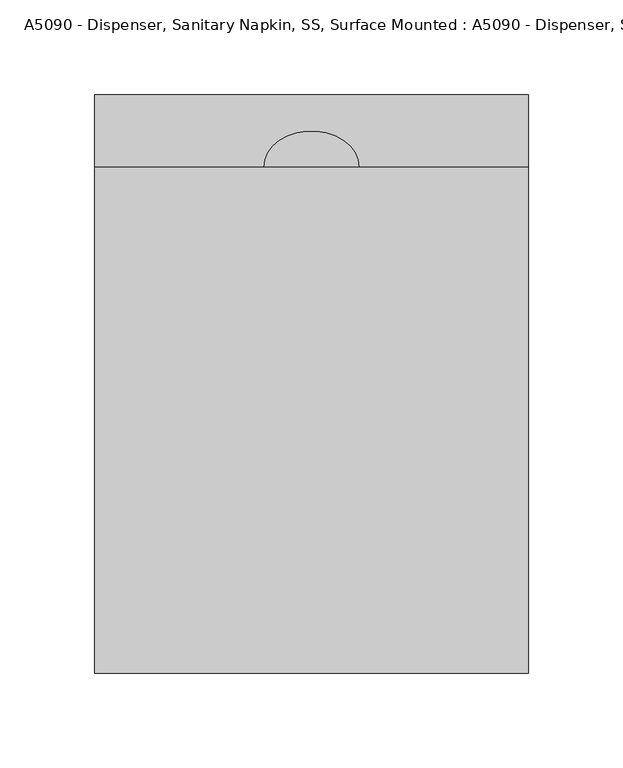
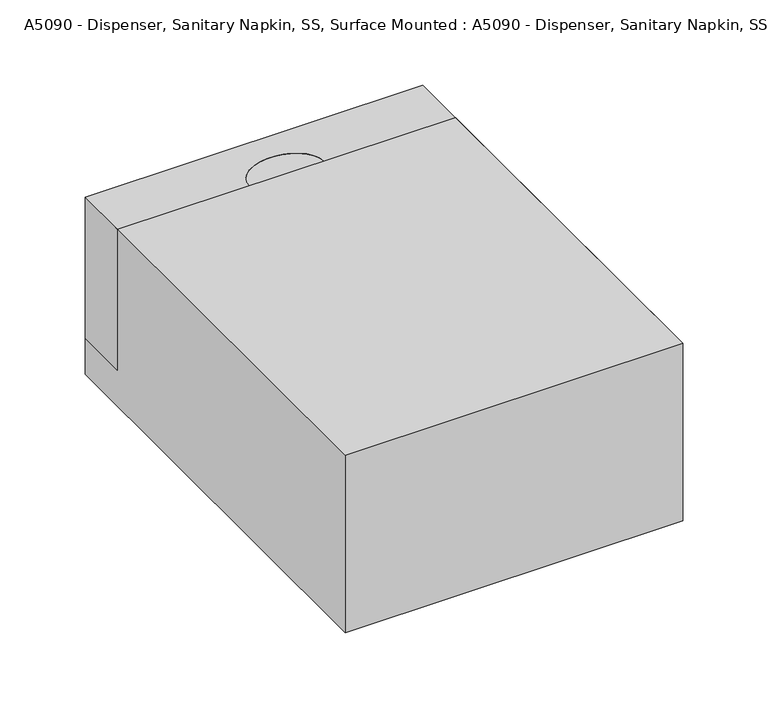
"""IFC4 building model written with IfcOpenShell, lengths in millimetres: proxy geometry, A5090 - Dispenser, Sanitary Napkin, SS, Surface Mounted : A5090 - Dispenser, Sanitary Napkin, SS, Surface Mounted."""

import ifcopenshell
import ifcopenshell.guid

model = None  # the IFC model being written
_history = None  # IfcOwnerHistory: only IFC2X3 demands one
_inside = {}  # id of a spatial element -> (the spatial element, [elements in it])
_under = {}  # id of a project, library or spatial element -> (it, [spatial elements below it])
_declared = {}  # id of a project -> (the project, [libraries it declares])
_typed = {}  # id of a type object -> (the type object, [elements of that type])
_made_of = {}  # id of a material, layer set ... -> (it, [elements and type objects made of it])


def new_model(schema):
    """Start an empty IFC model of exactly this schema.

    Asked for "IFC4X3", IfcOpenShell would pick the latest addendum, in which some entities
    have other attributes; the version numbers below select the first issue.
    IFC2X3 requires an IfcOwnerHistory on every rooted entity: one is made here for all.
    """
    global model, _history
    if schema == "IFC4X3":
        model = ifcopenshell.file(schema_version=(4, 3, 0, 0))
    else:
        model = ifcopenshell.file(schema=schema)
    _inside.clear()
    _under.clear()
    _declared.clear()
    _typed.clear()
    _made_of.clear()
    _history = None
    if model.schema == "IFC2X3":
        org = make("IfcOrganization", Name="unknown")
        user = make(
            "IfcPersonAndOrganization",
            ThePerson=make("IfcPerson", FamilyName="unknown"),
            TheOrganization=org,
        )
        app = make(
            "IfcApplication",
            ApplicationDeveloper=org,
            Version="unknown",
            ApplicationFullName="unknown",
            ApplicationIdentifier="unknown",
        )
        _history = make(
            "IfcOwnerHistory",
            OwningUser=user,
            OwningApplication=app,
            ChangeAction="ADDED",
            CreationDate=0,
        )
    return model


def make(cls, **values):
    """One entity of the class cls with the attributes given. An attribute that is None is left unset."""
    return model.create_entity(
        cls, **{name: value for name, value in values.items() if value is not None}
    )


def rooted(cls, **values):
    """An entity with a GlobalId (a new one), such as an element, a storey or a relation."""
    return make(cls, GlobalId=ifcopenshell.guid.new(), OwnerHistory=_history, **values)


def si_unit(unit_type, name, prefix=None):
    """IfcSIUnit, for example si_unit("LENGTHUNIT", "METRE", prefix="MILLI")."""
    return make("IfcSIUnit", UnitType=unit_type, Prefix=prefix, Name=name)


def assignment(units):
    """IfcUnitAssignment: the units of a project."""
    return None if units is None else make("IfcUnitAssignment", Units=units)


def point(xyz):
    """IfcCartesianPoint."""
    return None if xyz is None else make("IfcCartesianPoint", Coordinates=xyz)


def direction(xyz):
    """IfcDirection."""
    return None if xyz is None else make("IfcDirection", DirectionRatios=xyz)


def frame(location, z_axis=None, x_axis=None):
    """IfcAxis2Placement3D, a coordinate frame: its origin and axes. An axis left out is left unset."""
    return make(
        "IfcAxis2Placement3D",
        Location=point(location),
        Axis=direction(z_axis),
        RefDirection=direction(x_axis),
    )


def origin():
    """The frame at (0, 0, 0) with its axes left unset."""
    return frame((0.0, 0.0, 0.0))


def origin_with_axes():
    """The frame at (0, 0, 0) with the z axis (0, 0, 1) and the x axis (1, 0, 0) written out."""
    return frame((0.0, 0.0, 0.0), z_axis=(0.0, 0.0, 1.0), x_axis=(1.0, 0.0, 0.0))


def place(relative_to, where):
    """IfcLocalPlacement: puts the frame where relative to a parent placement (None: the world)."""
    return make(
        "IfcLocalPlacement", PlacementRelTo=relative_to, RelativePlacement=where
    )


def context(
    kind, dimensions, precision=None, world=None, true_north=None, identifier=None
):
    """IfcGeometricRepresentationContext, for example the 3D "Model" context."""
    return make(
        "IfcGeometricRepresentationContext",
        ContextIdentifier=identifier,
        ContextType=kind,
        CoordinateSpaceDimension=dimensions,
        Precision=precision,
        WorldCoordinateSystem=world,
        TrueNorth=true_north,
    )


def project(units=None, contexts=None):
    """IfcProject with its units and contexts."""
    return rooted(
        "IfcProject",
        Name="project",
        RepresentationContexts=contexts,
        UnitsInContext=assignment(units),
    )


def spatial(cls, under=None, at=None, **own):
    """A site, building, storey or space (cls), placed at a placement, below another one or the project."""
    s = rooted(cls, ObjectPlacement=at, **own)
    if under is not None:
        _under.setdefault(under.id(), (under, []))[1].append(s)
    return s


def polyline(points):
    """IfcPolyline through the points."""
    return make("IfcPolyline", Points=[point(p) for p in points])


def ellipse_curve(where, semi_axis1, semi_axis2):
    """IfcEllipse in the frame where."""
    return make(
        "IfcEllipse", Position=where, SemiAxis1=semi_axis1, SemiAxis2=semi_axis2
    )


def trimmed(basis, trim1, trim2, sense, master):
    """IfcTrimmedCurve: the piece of a basis curve between two trims."""
    return make(
        "IfcTrimmedCurve",
        BasisCurve=basis,
        Trim1=trim1,
        Trim2=trim2,
        SenseAgreement=sense,
        MasterRepresentation=master,
    )


def outline(outer, holes=None, kind="AREA"):
    """IfcArbitraryClosedProfileDef: a profile drawn as a closed curve; with holes, ...WithVoids."""
    if holes is None:
        return make("IfcArbitraryClosedProfileDef", ProfileType=kind, OuterCurve=outer)
    return make(
        "IfcArbitraryProfileDefWithVoids",
        ProfileType=kind,
        OuterCurve=outer,
        InnerCurves=holes,
    )


def extrude(swept, where, along, depth):
    """IfcExtrudedAreaSolid: the profile swept, set in the frame where, extruded along a direction by depth."""
    return make(
        "IfcExtrudedAreaSolid",
        SweptArea=swept,
        Position=where,
        ExtrudedDirection=direction(along),
        Depth=depth,
    )


def shape(context_of_items, identifier, shape_type, items):
    """IfcShapeRepresentation: the items that make up one representation, for example the "Body"."""
    return make(
        "IfcShapeRepresentation",
        ContextOfItems=context_of_items,
        RepresentationIdentifier=identifier,
        RepresentationType=shape_type,
        Items=items,
    )


def source(mapping_origin, context_of_items, identifier, shape_type, items):
    """IfcRepresentationMap: a shape defined once, which mapped items show again and again."""
    return make(
        "IfcRepresentationMap",
        MappingOrigin=mapping_origin,
        MappedRepresentation=shape(context_of_items, identifier, shape_type, items),
    )


def transform(
    local_origin,
    x_axis=None,
    y_axis=None,
    z_axis=None,
    scale=None,
    scale2=None,
    scale3=None,
    uniform=True,
):
    """IfcCartesianTransformationOperator3D, or its non-uniform kind. x_axis, y_axis, z_axis: its Axis1, 2, 3."""
    if uniform:
        return make(
            "IfcCartesianTransformationOperator3D",
            Axis1=direction(x_axis),
            Axis2=direction(y_axis),
            LocalOrigin=point(local_origin),
            Scale=scale,
            Axis3=direction(z_axis),
        )
    return make(
        "IfcCartesianTransformationOperator3DnonUniform",
        Axis1=direction(x_axis),
        Axis2=direction(y_axis),
        LocalOrigin=point(local_origin),
        Scale=scale,
        Axis3=direction(z_axis),
        Scale2=scale2,
        Scale3=scale3,
    )


def mapped(mapping_source, mapping_target):
    """IfcMappedItem: shows the shape of a source again, moved by a transform."""
    return make(
        "IfcMappedItem", MappingSource=mapping_source, MappingTarget=mapping_target
    )


def made_of(thing, what):
    """Note that an element or type object is made of a material, layer set ...; save() writes the relation."""
    if what is not None:
        _made_of.setdefault(what.id(), (what, []))[1].append(thing)
    return thing


def element(
    cls,
    number,
    at=None,
    inside=None,
    cuts=None,
    type_object=None,
    material=None,
    context=None,
    identifier="Body",
    shape_type=None,
    held_by="IfcProductDefinitionShape",
    body=None,
    shapes=None,
    **own,
):
    """One element of the class cls, such as IfcWall. Its Tag is "e" and its number.

    at: its placement. inside: the storey or other place that contains it. cuts: it is an
    opening in that element (IfcRelVoidsElement). A single representation is given by context,
    identifier, shape_type and body (its items); several are given by shapes. held_by: the class
    of the entity that holds the representations. save() writes the other relations.
    """
    e = rooted(cls, Tag="e%d" % number, ObjectPlacement=at, **own)
    if body is not None:
        shapes = [shape(context, identifier, shape_type, body)]
    if shapes is not None:
        e.Representation = make(held_by, Representations=shapes)
    if inside is not None:
        _inside.setdefault(inside.id(), (inside, []))[1].append(e)
    if cuts is not None:
        rooted(
            "IfcRelVoidsElement", RelatingBuildingElement=cuts, RelatedOpeningElement=e
        )
    if type_object is not None:
        _typed.setdefault(type_object.id(), (type_object, []))[1].append(e)
    return made_of(e, material)


def aggregate(whole, parts):
    """IfcRelAggregates: a whole, such as a stair, and the parts it consists of."""
    return rooted("IfcRelAggregates", RelatingObject=whole, RelatedObjects=parts)


def save(model, path):
    """Write the relations noted so far, then the file.

    IfcRelAggregates (storeys below a building ...), IfcRelContainedInSpatialStructure (elements
    in a storey), IfcRelDefinesByType, IfcRelAssociatesMaterial and IfcRelDeclares: one each for
    every whole, place, type object, material and project.
    """
    for whole, parts in _under.values():
        aggregate(whole, parts)
    for where, things in _inside.values():
        rooted(
            "IfcRelContainedInSpatialStructure",
            RelatedElements=things,
            RelatingStructure=where,
        )
    for kind, things in _typed.values():
        rooted("IfcRelDefinesByType", RelatedObjects=things, RelatingType=kind)
    for what, things in _made_of.values():
        rooted("IfcRelAssociatesMaterial", RelatedObjects=things, RelatingMaterial=what)
    for by, libraries in _declared.values():
        rooted("IfcRelDeclares", RelatingContext=by, RelatedDefinitions=libraries)
    model.write(path)


def plane_surface(at):
    """IfcPlane: the flat surface through the origin of the frame at, square to its z axis."""
    return make("IfcPlane", Position=at)


def extruded_surface(curve, direction_of_extrusion, depth):
    """IfcSurfaceOfLinearExtrusion: the curve pushed along a direction by depth."""
    return make(
        "IfcSurfaceOfLinearExtrusion",
        SweptCurve=make("IfcArbitraryOpenProfileDef", ProfileType="CURVE", Curve=curve),
        ExtrudedDirection=direction(direction_of_extrusion),
        Depth=depth,
    )


def advanced_brep(points, edges, surfaces, faces):
    """IfcAdvancedBrep: a solid bounded by faces that lie on surfaces and meet in shared edges.

    An edge is (start, end): straight between two places in points (the first is 0);
    or (start, end, curve); or (start, end, curve, False) where it runs against its curve.
    A face is (place in surfaces, loops), or (place, loops, False) where it looks against
    its surface's normal. A loop lists edges by number (the first is 1), with a minus sign
    where the edge is run from its end to its start. The first loop is the outer one.
    """
    corners = [point(p) for p in points]
    vertices = [make("IfcVertexPoint", VertexGeometry=c) for c in corners]
    made = []
    for start, end, *more in edges:
        made.append(
            make(
                "IfcEdgeCurve",
                EdgeStart=vertices[start],
                EdgeEnd=vertices[end],
                EdgeGeometry=more[0] if more else make("IfcPolyline", Points=[corners[start], corners[end]]),
                SameSense=more[1] if len(more) > 1 else True,
            )
        )
    hull = []
    for where, loops, *sense in faces:
        bounds = []
        for j, loop in enumerate(loops):
            ring = [make("IfcOrientedEdge", EdgeElement=made[abs(k) - 1], Orientation=k > 0) for k in loop]
            bounds.append(
                make(
                    "IfcFaceOuterBound" if j == 0 else "IfcFaceBound",
                    Bound=make("IfcEdgeLoop", EdgeList=ring),
                    Orientation=True,
                )
            )
        hull.append(make("IfcAdvancedFace", Bounds=bounds, FaceSurface=surfaces[where], SameSense=sense[0] if sense else True))
    return make("IfcAdvancedBrep", Outer=make("IfcClosedShell", CfsFaces=hull))


def a5090_dispenser_sanitary_napkin_ss_surface_mounted_a5090_ce8c1d57(model_context):
    return source(origin(), model_context, "Body", "SolidModel", [
        extrude(outline(polyline([(0.0, 127.0), (266.7, 127.0), (266.7, 25.4), (304.8, 25.4), (304.8, 0.0), (0.0, 0.0), (0.0, 127.0)])), frame((-114.3, 0.0, 0.0), z_axis=(1.0, 0.0, 0.0), x_axis=(0.0, 1.0, 0.0)), (0.0, 0.0, 1.0), 228.6),
        advanced_brep(
        [(114.3, 304.8, 127.0), (-114.3, 304.8, 127.0), (-114.3, 266.7, 127.0), (-25.4, 266.7, 127.0), (25.4, 266.7, 127.0), (114.3, 266.7, 127.0), (114.3, 304.8, 25.4), (114.3, 266.7, 25.4), (25.4, 266.7, 25.4), (-25.4, 266.7, 25.4), (-114.3, 266.7, 25.4), (-114.3, 304.8, 25.4)],
        [
            (0, 1),
            (1, 2),
            (2, 3),
            (3, 4, ellipse_curve(frame((0.0, 266.7, 127.0), z_axis=(0.0, 0.0, -1.0), x_axis=(1.0, 0.0, 0.0)), 25.4, 19.05)),
            (4, 5),
            (5, 0),
            (6, 7),
            (7, 8),
            (8, 9, ellipse_curve(frame((0.0, 266.7, 25.4), z_axis=(0.0, 0.0, 1.0), x_axis=(1.0, 0.0, 0.0)), 25.4, 19.05)),
            (9, 10),
            (10, 11),
            (11, 6),
            (0, 6),
            (11, 1),
            (10, 2),
            (9, 3),
            (8, 4),
            (7, 5),
        ],
        [
            plane_surface(frame((-114.3, 304.8, 127.0), z_axis=(0.0, 0.0, 1.0), x_axis=(-1.0, 0.0, 0.0))),
            plane_surface(frame((-114.3, 304.8, 25.4), z_axis=(0.0, 0.0, -1.0), x_axis=(1.0, 0.0, 0.0))),
            plane_surface(frame((114.3, 304.8, 127.0), z_axis=(0.0, 1.0, 0.0), x_axis=(0.0, 0.0, -1.0))),
            plane_surface(frame((-114.3, 304.8, 127.0), z_axis=(-1.0, 0.0, 0.0), x_axis=(0.0, 0.0, -1.0))),
            plane_surface(frame((-114.3, 266.7, 127.0), z_axis=(0.0, -1.0, 0.0), x_axis=(0.0, 0.0, -1.0))),
            extruded_surface(trimmed(ellipse_curve(frame((0.0, 266.7, -76.2), z_axis=(0.0, 0.0, -1.0), x_axis=(1.0, 0.0, 0.0)), 25.4, 19.05), [point((-25.4, 266.7, -76.2))], [point((25.4, 266.7, -76.2))], True, "CARTESIAN"), (0.0, 0.0, 101.6), 101.6),
            plane_surface(frame((25.4, 266.7, 127.0), z_axis=(0.0, -1.0, 0.0), x_axis=(0.0, 0.0, -1.0))),
            plane_surface(frame((114.3, 266.7, 127.0), z_axis=(1.0, 0.0, 0.0), x_axis=(0.0, 0.0, -1.0))),
        ],
        [
            (0, [[1, 2, 3, 4, 5, 6]]),
            (1, [[7, 8, 9, 10, 11, 12]]),
            (2, [[-1, 13, -12, 14]]),
            (3, [[-2, -14, -11, 15]]),
            (4, [[-3, -15, -10, 16]]),
            (5, [[-4, -16, -9, 17]]),
            (6, [[-5, -17, -8, 18]]),
            (7, [[-6, -18, -7, -13]]),
        ],
    ),
        extrude(outline(polyline([(114.3, 304.8), (114.3, 0.0), (-114.3, 0.0), (-114.3, 304.8), (114.3, 304.8)])), origin_with_axes(), (0.0, 0.0, 1.0), 127.0),
    ])


if __name__ == "__main__":
    model = new_model("IFC4")
    model_context = context("Model", 3, world=origin())
    ifc_project = project(units=[si_unit("LENGTHUNIT", "METRE", prefix="MILLI")], contexts=[model_context])
    site = spatial("IfcSite", under=ifc_project)
    building = spatial("IfcBuilding", under=site)
    placement = place(None, origin())
    a5090_dispenser_sanitary_napkin_ss_surface_mounted_a5090_shape = a5090_dispenser_sanitary_napkin_ss_surface_mounted_a5090_ce8c1d57(model_context)
    element("IfcBuildingElementProxy", 1, Name="A5090 - Dispenser, Sanitary Napkin, SS, Surface Mounted : A5090 - Dispenser, Sanitary Napkin, SS, Surface Mounted", ObjectType="A5090 - Dispenser, Sanitary Napkin, SS, Surface Mounted : A5090 - Dispenser, Sanitary Napkin, SS, Surface Mounted", at=placement, inside=building, context=model_context, shape_type="MappedRepresentation", body=[
        mapped(a5090_dispenser_sanitary_napkin_ss_surface_mounted_a5090_shape, transform((0.0, 0.0, 0.0), x_axis=(1.0, 0.0, 0.0), y_axis=(0.0, 1.0, 0.0), z_axis=(0.0, 0.0, 1.0))),
    ])
    save(model, "model.ifc")

# Revit data of these elements
# Type "A5090 - Dispenser, Sanitary Napkin, SS, Surface Mounted : A5090 - Dispenser, Sanitary Napkin, SS, Surface Mounted"
#   Watts2 = "0"
#   Watts1 = "0"
#   Unit_Issue = "EA"
#   UTIL_6_Misc = "-"
#   UTIL_5_NonMedGas = "-"
#   UTIL_4_MiscGas = "-"
#   UTIL_3_MedGas = "-"
#   UTIL_2_Elec = "-"
#   UTIL_1_WaterDrain = "-"
#   Nomenclature = "Disposal, Sanitary Napkin, SS, Surface Mounted"
#   NSN = "7240"
#   Location [instance default] = ""
#   JSN = "A5090"
#   Fund_Source_VA = "-"
#   Fund_Source_Navy = "-"
#   Fund_Source_Army = "-"
#   Fund_Source_AF = "-"
#   ELEC_Volts2 = "0"
#   ELEC_Volts1 = "0"
#   ELEC_Phase2 = "0"
#   ELEC_Phase1 = "0"
#   ELEC_HertzSwitch = "0"
#   ELEC_HertzDependent = "0"
#   ELEC_Hertz = "0"
#   ELEC_Amps2 = "0"
#   ELEC_Amps1 = "0"
#   DetailDescription = "A surface mounted, satin finish stainless steel, sanitary napkin disposal. Disposal features a flip-up cover, secured to the container by a heavy duty stainless steel piano-hinge. Disposal may be secured to wall or toilet partition. For general purpose use in female toilet stalls or rooms and uni-sex toilet rooms."
#   CAT_VA = "A"
#   CAT_Navy = "A"
#   CAT_IHS = "-"
#   CAT_Army = "A"
#   CAT_AF = "A"
#   BTUperhour = "0"
#   Weight_IP = 4
#   Default Elevation = 1' - 0"
#   DIM_Width_IP = 0' - 9"
#   DIM_Height_IP = 1' - 0"
#   DIM_Depth_IP = 0' - 5"
#   Assembly Code = ""
# Element 1 (IfcBuildingElementProxy, "A5090 - Dispenser, Sanitary Napkin, SS, Surface Mounted : A5090 - Dispenser, Sanitary Napkin, SS, Surface Mounted")
#   Location = "TLTU1"
#   Materials on its faces: "EquipSpace"
# Materials
#   "EquipSpace": class "Unassigned", colour RGB 221 217 195, transparency 0.5
